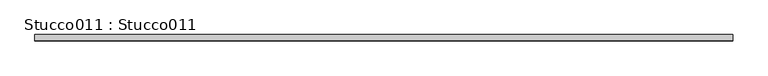
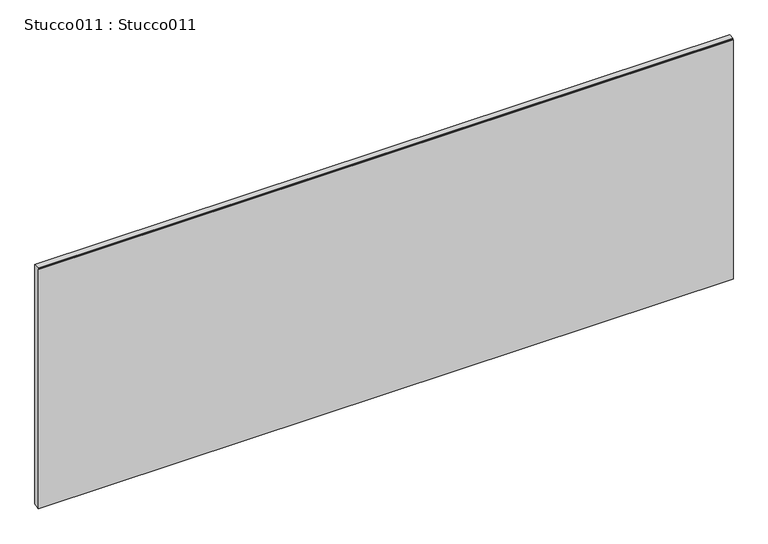
"""IFC4 building model written with IfcOpenShell, lengths in millimetres: proxy geometry, Stucco011 : Stucco011."""

from ifc_helpers import new_model, si_unit, frame, origin, place, context, project, spatial, polyline, outline, extrude, source, transform, mapped, element, save


def stucco011_stucco011_0b6d7d4c(model_context):
    return source(origin(), model_context, "Body", "SweptSolid", [
        extrude(outline(polyline([(-4434.3425368, 40306.7927615), (-4434.3425368, 41036.7712), (-4433.0725368, 41036.7712), (-4433.0725368, 41040.251), (-4416.5625, 41040.251), (-4416.5625, 40312.5195313), (-4434.3425368, 40306.7927615)])), frame((12383.0178845, 0.0, 0.0), z_axis=(1.0, 0.0, 0.0), x_axis=(0.0, 1.0, 0.0)), (0.0, 0.0, 1.0), 2000.0),
    ])


if __name__ == "__main__":
    model = new_model("IFC4")
    model_context = context("Model", 3, world=origin())
    ifc_project = project(units=[si_unit("LENGTHUNIT", "METRE", prefix="MILLI")], contexts=[model_context])
    site = spatial("IfcSite", under=ifc_project)
    building = spatial("IfcBuilding", under=site)
    placement = place(None, origin())
    stucco011_stucco011_shape = stucco011_stucco011_0b6d7d4c(model_context)
    element("IfcBuildingElementProxy", 1, Name="Stucco011 : Stucco011", ObjectType="Stucco011 : Stucco011", at=placement, inside=building, context=model_context, shape_type="MappedRepresentation", body=[
        mapped(stucco011_stucco011_shape, transform((0.0, 0.0, 0.0), x_axis=(1.0, 0.0, 0.0), y_axis=(0.0, 1.0, 0.0), z_axis=(0.0, 0.0, 1.0))),
    ])
    save(model, "model.ifc")

# Revit data of these elements
# Type "Stucco011 : Stucco011"
#   NameOverride = "Stucco011"
# Element 1 (IfcBuildingElementProxy, "Stucco011 : Stucco011")
#   Materials on its faces: "7/8\" SMOOTH TROWEL EXTERIOR STUCCO"
# Materials
#   "7/8\" SMOOTH TROWEL EXTERIOR STUCCO": class "Unassigned", colour RGB 255 255 255, transparency 0, Cost = 0
